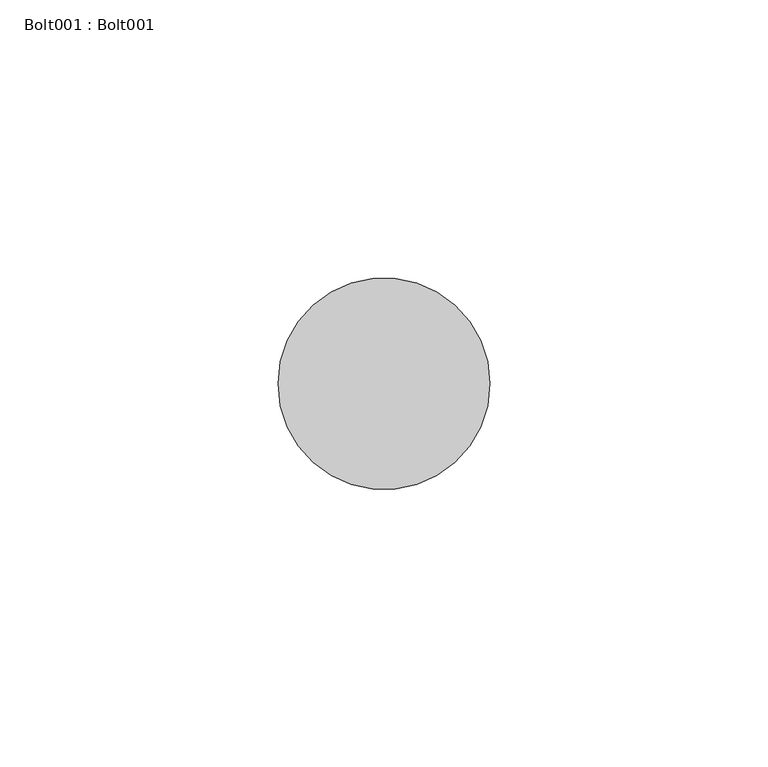
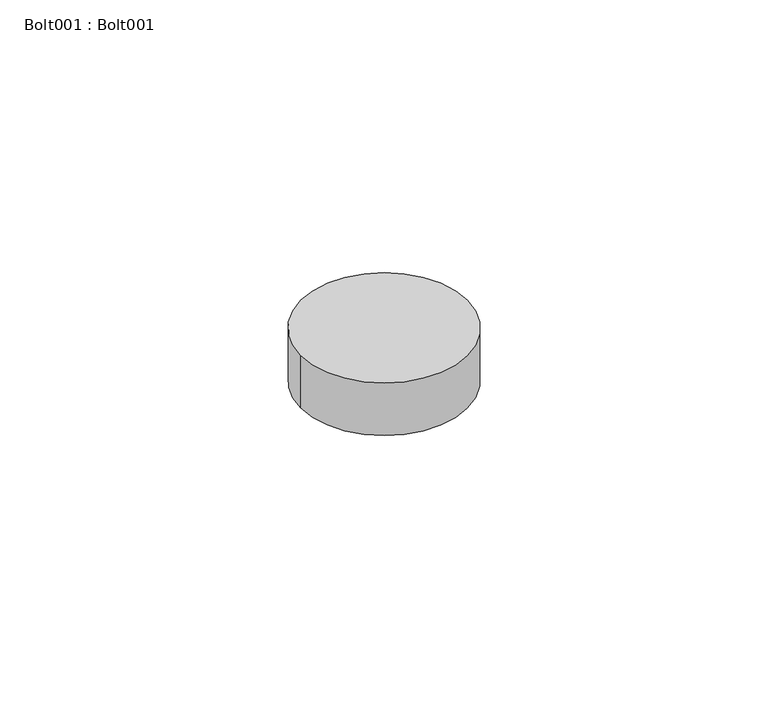
"""IFC4 building model written with IfcOpenShell, lengths in millimetres: proxy geometry, Bolt001 : Bolt001."""

import ifcopenshell
import ifcopenshell.guid

model = None  # the IFC model being written
_history = None  # IfcOwnerHistory: only IFC2X3 demands one
_inside = {}  # id of a spatial element -> (the spatial element, [elements in it])
_under = {}  # id of a project, library or spatial element -> (it, [spatial elements below it])
_declared = {}  # id of a project -> (the project, [libraries it declares])
_typed = {}  # id of a type object -> (the type object, [elements of that type])
_made_of = {}  # id of a material, layer set ... -> (it, [elements and type objects made of it])


def new_model(schema):
    """Start an empty IFC model of exactly this schema.

    Asked for "IFC4X3", IfcOpenShell would pick the latest addendum, in which some entities
    have other attributes; the version numbers below select the first issue.
    IFC2X3 requires an IfcOwnerHistory on every rooted entity: one is made here for all.
    """
    global model, _history
    if schema == "IFC4X3":
        model = ifcopenshell.file(schema_version=(4, 3, 0, 0))
    else:
        model = ifcopenshell.file(schema=schema)
    _inside.clear()
    _under.clear()
    _declared.clear()
    _typed.clear()
    _made_of.clear()
    _history = None
    if model.schema == "IFC2X3":
        org = make("IfcOrganization", Name="unknown")
        user = make(
            "IfcPersonAndOrganization",
            ThePerson=make("IfcPerson", FamilyName="unknown"),
            TheOrganization=org,
        )
        app = make(
            "IfcApplication",
            ApplicationDeveloper=org,
            Version="unknown",
            ApplicationFullName="unknown",
            ApplicationIdentifier="unknown",
        )
        _history = make(
            "IfcOwnerHistory",
            OwningUser=user,
            OwningApplication=app,
            ChangeAction="ADDED",
            CreationDate=0,
        )
    return model


def make(cls, **values):
    """One entity of the class cls with the attributes given. An attribute that is None is left unset."""
    return model.create_entity(
        cls, **{name: value for name, value in values.items() if value is not None}
    )


def rooted(cls, **values):
    """An entity with a GlobalId (a new one), such as an element, a storey or a relation."""
    return make(cls, GlobalId=ifcopenshell.guid.new(), OwnerHistory=_history, **values)


def si_unit(unit_type, name, prefix=None):
    """IfcSIUnit, for example si_unit("LENGTHUNIT", "METRE", prefix="MILLI")."""
    return make("IfcSIUnit", UnitType=unit_type, Prefix=prefix, Name=name)


def assignment(units):
    """IfcUnitAssignment: the units of a project."""
    return None if units is None else make("IfcUnitAssignment", Units=units)


def point(xyz):
    """IfcCartesianPoint."""
    return None if xyz is None else make("IfcCartesianPoint", Coordinates=xyz)


def direction(xyz):
    """IfcDirection."""
    return None if xyz is None else make("IfcDirection", DirectionRatios=xyz)


def frame(location, z_axis=None, x_axis=None):
    """IfcAxis2Placement3D, a coordinate frame: its origin and axes. An axis left out is left unset."""
    return make(
        "IfcAxis2Placement3D",
        Location=point(location),
        Axis=direction(z_axis),
        RefDirection=direction(x_axis),
    )


def frame_2d(location, x_axis=None):
    """IfcAxis2Placement2D, a coordinate frame in the plane: its origin and x axis."""
    return make(
        "IfcAxis2Placement2D", Location=point(location), RefDirection=direction(x_axis)
    )


def origin():
    """The frame at (0, 0, 0) with its axes left unset."""
    return frame((0.0, 0.0, 0.0))


def place(relative_to, where):
    """IfcLocalPlacement: puts the frame where relative to a parent placement (None: the world)."""
    return make(
        "IfcLocalPlacement", PlacementRelTo=relative_to, RelativePlacement=where
    )


def context(
    kind, dimensions, precision=None, world=None, true_north=None, identifier=None
):
    """IfcGeometricRepresentationContext, for example the 3D "Model" context."""
    return make(
        "IfcGeometricRepresentationContext",
        ContextIdentifier=identifier,
        ContextType=kind,
        CoordinateSpaceDimension=dimensions,
        Precision=precision,
        WorldCoordinateSystem=world,
        TrueNorth=true_north,
    )


def project(units=None, contexts=None):
    """IfcProject with its units and contexts."""
    return rooted(
        "IfcProject",
        Name="project",
        RepresentationContexts=contexts,
        UnitsInContext=assignment(units),
    )


def spatial(cls, under=None, at=None, **own):
    """A site, building, storey or space (cls), placed at a placement, below another one or the project."""
    s = rooted(cls, ObjectPlacement=at, **own)
    if under is not None:
        _under.setdefault(under.id(), (under, []))[1].append(s)
    return s


def circle_curve(where, radius):
    """IfcCircle in the frame where."""
    return make("IfcCircle", Position=where, Radius=radius)


def trimmed(basis, trim1, trim2, sense, master):
    """IfcTrimmedCurve: the piece of a basis curve between two trims."""
    return make(
        "IfcTrimmedCurve",
        BasisCurve=basis,
        Trim1=trim1,
        Trim2=trim2,
        SenseAgreement=sense,
        MasterRepresentation=master,
    )


def segment(curve, same_sense, transition):
    """IfcCompositeCurveSegment."""
    return make(
        "IfcCompositeCurveSegment",
        Transition=transition,
        SameSense=same_sense,
        ParentCurve=curve,
    )


def composite_curve(segments, self_intersect=None):
    """IfcCompositeCurve: segments joined end to end."""
    return make("IfcCompositeCurve", Segments=segments, SelfIntersect=self_intersect)


def outline(outer, holes=None, kind="AREA"):
    """IfcArbitraryClosedProfileDef: a profile drawn as a closed curve; with holes, ...WithVoids."""
    if holes is None:
        return make("IfcArbitraryClosedProfileDef", ProfileType=kind, OuterCurve=outer)
    return make(
        "IfcArbitraryProfileDefWithVoids",
        ProfileType=kind,
        OuterCurve=outer,
        InnerCurves=holes,
    )


def extrude(swept, where, along, depth):
    """IfcExtrudedAreaSolid: the profile swept, set in the frame where, extruded along a direction by depth."""
    return make(
        "IfcExtrudedAreaSolid",
        SweptArea=swept,
        Position=where,
        ExtrudedDirection=direction(along),
        Depth=depth,
    )


def shape(context_of_items, identifier, shape_type, items):
    """IfcShapeRepresentation: the items that make up one representation, for example the "Body"."""
    return make(
        "IfcShapeRepresentation",
        ContextOfItems=context_of_items,
        RepresentationIdentifier=identifier,
        RepresentationType=shape_type,
        Items=items,
    )


def source(mapping_origin, context_of_items, identifier, shape_type, items):
    """IfcRepresentationMap: a shape defined once, which mapped items show again and again."""
    return make(
        "IfcRepresentationMap",
        MappingOrigin=mapping_origin,
        MappedRepresentation=shape(context_of_items, identifier, shape_type, items),
    )


def transform(
    local_origin,
    x_axis=None,
    y_axis=None,
    z_axis=None,
    scale=None,
    scale2=None,
    scale3=None,
    uniform=True,
):
    """IfcCartesianTransformationOperator3D, or its non-uniform kind. x_axis, y_axis, z_axis: its Axis1, 2, 3."""
    if uniform:
        return make(
            "IfcCartesianTransformationOperator3D",
            Axis1=direction(x_axis),
            Axis2=direction(y_axis),
            LocalOrigin=point(local_origin),
            Scale=scale,
            Axis3=direction(z_axis),
        )
    return make(
        "IfcCartesianTransformationOperator3DnonUniform",
        Axis1=direction(x_axis),
        Axis2=direction(y_axis),
        LocalOrigin=point(local_origin),
        Scale=scale,
        Axis3=direction(z_axis),
        Scale2=scale2,
        Scale3=scale3,
    )


def mapped(mapping_source, mapping_target):
    """IfcMappedItem: shows the shape of a source again, moved by a transform."""
    return make(
        "IfcMappedItem", MappingSource=mapping_source, MappingTarget=mapping_target
    )


def made_of(thing, what):
    """Note that an element or type object is made of a material, layer set ...; save() writes the relation."""
    if what is not None:
        _made_of.setdefault(what.id(), (what, []))[1].append(thing)
    return thing


def element(
    cls,
    number,
    at=None,
    inside=None,
    cuts=None,
    type_object=None,
    material=None,
    context=None,
    identifier="Body",
    shape_type=None,
    held_by="IfcProductDefinitionShape",
    body=None,
    shapes=None,
    **own,
):
    """One element of the class cls, such as IfcWall. Its Tag is "e" and its number.

    at: its placement. inside: the storey or other place that contains it. cuts: it is an
    opening in that element (IfcRelVoidsElement). A single representation is given by context,
    identifier, shape_type and body (its items); several are given by shapes. held_by: the class
    of the entity that holds the representations. save() writes the other relations.
    """
    e = rooted(cls, Tag="e%d" % number, ObjectPlacement=at, **own)
    if body is not None:
        shapes = [shape(context, identifier, shape_type, body)]
    if shapes is not None:
        e.Representation = make(held_by, Representations=shapes)
    if inside is not None:
        _inside.setdefault(inside.id(), (inside, []))[1].append(e)
    if cuts is not None:
        rooted(
            "IfcRelVoidsElement", RelatingBuildingElement=cuts, RelatedOpeningElement=e
        )
    if type_object is not None:
        _typed.setdefault(type_object.id(), (type_object, []))[1].append(e)
    return made_of(e, material)


def aggregate(whole, parts):
    """IfcRelAggregates: a whole, such as a stair, and the parts it consists of."""
    return rooted("IfcRelAggregates", RelatingObject=whole, RelatedObjects=parts)


def save(model, path):
    """Write the relations noted so far, then the file.

    IfcRelAggregates (storeys below a building ...), IfcRelContainedInSpatialStructure (elements
    in a storey), IfcRelDefinesByType, IfcRelAssociatesMaterial and IfcRelDeclares: one each for
    every whole, place, type object, material and project.
    """
    for whole, parts in _under.values():
        aggregate(whole, parts)
    for where, things in _inside.values():
        rooted(
            "IfcRelContainedInSpatialStructure",
            RelatedElements=things,
            RelatingStructure=where,
        )
    for kind, things in _typed.values():
        rooted("IfcRelDefinesByType", RelatedObjects=things, RelatingType=kind)
    for what, things in _made_of.values():
        rooted("IfcRelAssociatesMaterial", RelatedObjects=things, RelatingMaterial=what)
    for by, libraries in _declared.values():
        rooted("IfcRelDeclares", RelatingContext=by, RelatedDefinitions=libraries)
    model.write(path)


def bolt001_bolt001_70c8ac4d(model_context):
    return source(origin(), model_context, "Body", "SweptSolid", [
        extrude(outline(composite_curve([segment(trimmed(circle_curve(frame_2d((7251.9702148, -1781.8449707)), 19.05), [point((7232.9202148, -1781.8449707))], [point((7271.0202148, -1781.8449707))], False, "CARTESIAN"), True, "CONTINUOUS"), segment(trimmed(circle_curve(frame_2d((7251.9702148, -1781.8449707)), 19.05), [point((7271.0202148, -1781.8449707))], [point((7232.9202148, -1781.8449707))], False, "CARTESIAN"), True, "CONTINUOUS")], self_intersect=False)), frame((0.0, 0.0, 40112.696), z_axis=(0.0, 0.0, 1.0), x_axis=(1.0, 0.0, 0.0)), (0.0, 0.0, 1.0), 12.7),
    ])


if __name__ == "__main__":
    model = new_model("IFC4")
    model_context = context("Model", 3, world=origin())
    ifc_project = project(units=[si_unit("LENGTHUNIT", "METRE", prefix="MILLI")], contexts=[model_context])
    site = spatial("IfcSite", under=ifc_project)
    building = spatial("IfcBuilding", under=site)
    placement = place(None, origin())
    bolt001_bolt001_shape = bolt001_bolt001_70c8ac4d(model_context)
    element("IfcBuildingElementProxy", 1, Name="Bolt001 : Bolt001", ObjectType="Bolt001 : Bolt001", at=placement, inside=building, context=model_context, shape_type="MappedRepresentation", body=[
        mapped(bolt001_bolt001_shape, transform((0.0, 0.0, 0.0), x_axis=(1.0, 0.0, 0.0), y_axis=(0.0, 1.0, 0.0), z_axis=(0.0, 0.0, 1.0))),
    ])
    save(model, "model.ifc")

# Revit data of these elements
# Type "Bolt001 : Bolt001"
#   NameOverride = "Bolt001"
# Element 1 (IfcBuildingElementProxy, "Bolt001 : Bolt001")
#   Materials on its faces: "BOLTS CONCEALED BY FLOOR FINISH"
# Materials
#   "BOLTS CONCEALED BY FLOOR FINISH": class "Unassigned", colour RGB 128 128 128, transparency 0
